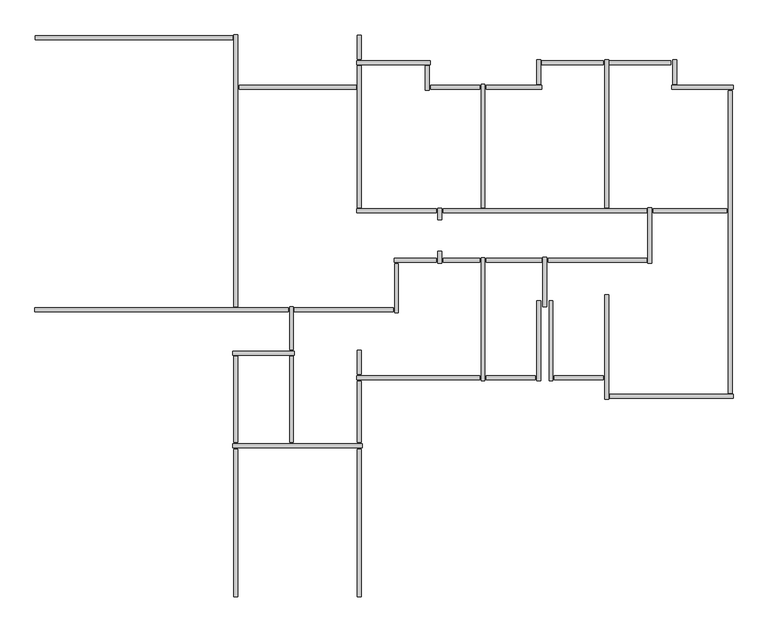
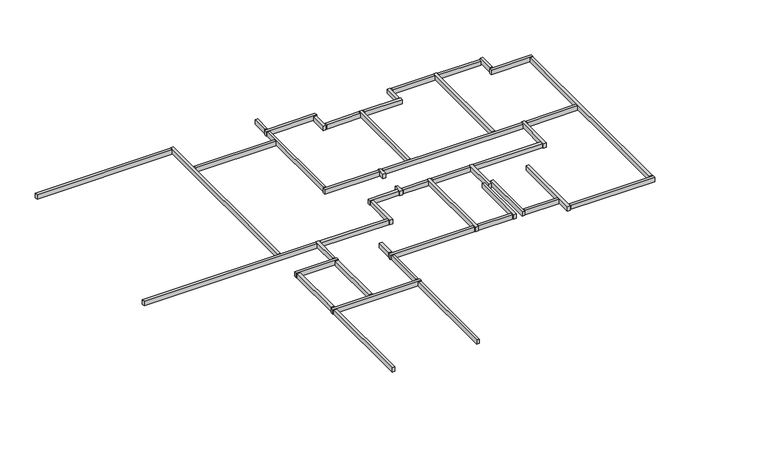
"""IFC4 building model written with IfcOpenShell, lengths in millimetres: beam geometry, Graute viga de respaldo1 : Graute viga de respaldo."""

from ifc_helpers import new_model, si_unit, frame, origin, place, context, project, spatial, polyline, outline, extrude, source, transform, mapped, element, save


def beam_8978719d(model_context):
    return source(origin(), model_context, "Body", "SweptSolid", [
        extrude(outline(polyline([(-62804.9587292, 72814.9577736), (-62804.9587292, 72720.9577736), (-67594.9587292, 72720.9577736), (-67594.9587292, 72814.9577736), (-62804.9587292, 72814.9577736)])), frame((0.0, 0.0, 2632.9999999), z_axis=(0.0, 0.0, 1.0), x_axis=(1.0, 0.0, 0.0)), (0.0, 0.0, 1.0), 167.0),
        extrude(outline(polyline([(-59771.9587292, 62785.4278788), (-59677.9587292, 62785.4278788), (-59677.9587292, 59195.4278788), (-59771.9587292, 59195.4278788), (-59771.9587292, 62785.4278788)])), frame((0.0, 0.0, 2632.9999999), z_axis=(0.0, 0.0, 1.0), x_axis=(1.0, 0.0, 0.0)), (0.0, 0.0, 1.0), 167.0),
        extrude(outline(polyline([(-62771.9587292, 62785.4278788), (-62677.9587292, 62785.4278788), (-62677.9587292, 59195.4278788), (-62771.9587292, 59195.4278788), (-62771.9587292, 62785.4278788)])), frame((0.0, 0.0, 2632.9999999), z_axis=(0.0, 0.0, 1.0), x_axis=(1.0, 0.0, 0.0)), (0.0, 0.0, 1.0), 167.0),
        extrude(outline(polyline([(-54994.9587292, 64468.4278788), (-54994.9587292, 64562.4278788), (-53804.9587292, 64562.4278788), (-53804.9587292, 64468.4278788), (-54994.9587292, 64468.4278788)])), frame((0.0, 0.0, 2632.9999999), z_axis=(0.0, 0.0, 1.0), x_axis=(1.0, 0.0, 0.0)), (0.0, 0.0, 1.0), 167.0),
        extrude(outline(polyline([(-56644.9587292, 64468.4278788), (-56644.9587292, 64562.4278788), (-55454.9587292, 64562.4278788), (-55454.9587292, 64468.4278788), (-56644.9587292, 64468.4278788)])), frame((0.0, 0.0, 2632.9999999), z_axis=(0.0, 0.0, 1.0), x_axis=(1.0, 0.0, 0.0)), (0.0, 0.0, 1.0), 167.0),
        extrude(outline(polyline([(-52594.9587292, 68518.4278788), (-52594.9587292, 68612.4278788), (-50804.9587292, 68612.4278788), (-50804.9587292, 68518.4278788), (-52594.9587292, 68518.4278788)])), frame((0.0, 0.0, 2632.9999999), z_axis=(0.0, 0.0, 1.0), x_axis=(1.0, 0.0, 0.0)), (0.0, 0.0, 1.0), 167.0),
        extrude(outline(polyline([(-57994.9587292, 71518.4278788), (-57994.9587292, 71612.4278788), (-56804.9587292, 71612.4278788), (-56804.9587292, 71518.4278788), (-57994.9587292, 71518.4278788)])), frame((0.0, 0.0, 2632.9999999), z_axis=(0.0, 0.0, 1.0), x_axis=(1.0, 0.0, 0.0)), (0.0, 0.0, 1.0), 167.0),
        extrude(outline(polyline([(-58027.9587292, 71495.4278788), (-58121.9587292, 71495.4278788), (-58121.9587292, 72085.4278788), (-58027.9587292, 72085.4278788), (-58027.9587292, 71495.4278788)])), frame((0.0, 0.0, 2632.9999999), z_axis=(0.0, 0.0, 1.0), x_axis=(1.0, 0.0, 0.0)), (0.0, 0.0, 1.0), 167.0),
        extrude(outline(polyline([(-59794.9587292, 72118.4278788), (-59794.9587292, 72212.4278788), (-58004.9587292, 72212.4278788), (-58004.9587292, 72118.4278788), (-59794.9587292, 72118.4278788)])), frame((0.0, 0.0, 2632.9999999), z_axis=(0.0, 0.0, 1.0), x_axis=(1.0, 0.0, 0.0)), (0.0, 0.0, 1.0), 167.0),
        extrude(outline(polyline([(-57821.9587292, 68635.4278788), (-57727.9587292, 68635.4278788), (-57727.9587292, 68345.4278788), (-57821.9587292, 68345.4278788), (-57821.9587292, 68635.4278788)])), frame((0.0, 0.0, 2632.9999999), z_axis=(0.0, 0.0, 1.0), x_axis=(1.0, 0.0, 0.0)), (0.0, 0.0, 1.0), 167.0),
        extrude(outline(polyline([(-55144.9587292, 67318.4278788), (-55144.9587292, 67412.4278788), (-52754.9587292, 67412.4278788), (-52754.9587292, 67318.4278788), (-55144.9587292, 67318.4278788)])), frame((0.0, 0.0, 2632.9999999), z_axis=(0.0, 0.0, 1.0), x_axis=(1.0, 0.0, 0.0)), (0.0, 0.0, 1.0), 167.0),
        extrude(outline(polyline([(-56644.9587292, 67318.4278788), (-56644.9587292, 67412.4278788), (-55304.9587292, 67412.4278788), (-55304.9587292, 67318.4278788), (-56644.9587292, 67318.4278788)])), frame((0.0, 0.0, 2632.9999999), z_axis=(0.0, 0.0, 1.0), x_axis=(1.0, 0.0, 0.0)), (0.0, 0.0, 1.0), 167.0),
        extrude(outline(polyline([(-57694.9587292, 67318.4278788), (-57694.9587292, 67412.4278788), (-56804.9587292, 67412.4278788), (-56804.9587292, 67318.4278788), (-57694.9587292, 67318.4278788)])), frame((0.0, 0.0, 2632.9999999), z_axis=(0.0, 0.0, 1.0), x_axis=(1.0, 0.0, 0.0)), (0.0, 0.0, 1.0), 167.0),
        extrude(outline(polyline([(-57821.9587292, 67585.4278788), (-57727.9587292, 67585.4278788), (-57727.9587292, 67295.4278788), (-57821.9587292, 67295.4278788), (-57821.9587292, 67585.4278788)])), frame((0.0, 0.0, 2632.9999999), z_axis=(0.0, 0.0, 1.0), x_axis=(1.0, 0.0, 0.0)), (0.0, 0.0, 1.0), 167.0),
        extrude(outline(polyline([(-58884.9587292, 67318.4278788), (-58884.9587292, 67412.4278788), (-57854.9587292, 67412.4278788), (-57854.9587292, 67318.4278788), (-58884.9587292, 67318.4278788)])), frame((0.0, 0.0, 2632.9999999), z_axis=(0.0, 0.0, 1.0), x_axis=(1.0, 0.0, 0.0)), (0.0, 0.0, 1.0), 167.0),
        extrude(outline(polyline([(-58777.9587292, 66095.4278788), (-58871.9587292, 66095.4278788), (-58871.9587292, 67285.4278788), (-58777.9587292, 67285.4278788), (-58777.9587292, 66095.4278788)])), frame((0.0, 0.0, 2632.9999999), z_axis=(0.0, 0.0, 1.0), x_axis=(1.0, 0.0, 0.0)), (0.0, 0.0, 1.0), 167.0),
        extrude(outline(polyline([(-61304.9587292, 66118.4278788), (-61304.9587292, 66212.4278788), (-58904.9587292, 66212.4278788), (-58904.9587292, 66118.4278788), (-61304.9587292, 66118.4278788)])), frame((0.0, 0.0, 2632.9999999), z_axis=(0.0, 0.0, 1.0), x_axis=(1.0, 0.0, 0.0)), (0.0, 0.0, 1.0), 167.0),
        extrude(outline(polyline([(-56771.9587292, 67430.4278788), (-56677.9587292, 67430.4278788), (-56677.9587292, 64445.4278788), (-56771.9587292, 64445.4278788), (-56771.9587292, 67430.4278788)])), frame((0.0, 0.0, 2632.9999999), z_axis=(0.0, 0.0, 1.0), x_axis=(1.0, 0.0, 0.0)), (0.0, 0.0, 1.0), 167.0),
        extrude(outline(polyline([(-59794.9587292, 64468.4278788), (-59794.9587292, 64562.4278788), (-56804.9587292, 64562.4278788), (-56804.9587292, 64468.4278788), (-59794.9587292, 64468.4278788)])), frame((0.0, 0.0, 2632.9999999), z_axis=(0.0, 0.0, 1.0), x_axis=(1.0, 0.0, 0.0)), (0.0, 0.0, 1.0), 167.0),
        extrude(outline(polyline([(-59771.9587292, 65185.4278788), (-59677.9587292, 65185.4278788), (-59677.9587292, 64595.4278788), (-59771.9587292, 64595.4278788), (-59771.9587292, 65185.4278788)])), frame((0.0, 0.0, 2632.9999999), z_axis=(0.0, 0.0, 1.0), x_axis=(1.0, 0.0, 0.0)), (0.0, 0.0, 1.0), 167.0),
        extrude(outline(polyline([(-59677.9587292, 62945.4278788), (-59771.9587292, 62945.4278788), (-59771.9587292, 64435.4278788), (-59677.9587292, 64435.4278788), (-59677.9587292, 62945.4278788)])), frame((0.0, 0.0, 2632.9999999), z_axis=(0.0, 0.0, 1.0), x_axis=(1.0, 0.0, 0.0)), (0.0, 0.0, 1.0), 167.0),
        extrude(outline(polyline([(-62677.9587292, 62945.4278788), (-62771.9587292, 62945.4278788), (-62771.9587292, 65035.4278788), (-62677.9587292, 65035.4278788), (-62677.9587292, 62945.4278788)])), frame((0.0, 0.0, 2632.9999999), z_axis=(0.0, 0.0, 1.0), x_axis=(1.0, 0.0, 0.0)), (0.0, 0.0, 1.0), 167.0),
        extrude(outline(polyline([(-61327.9587292, 62945.4278788), (-61421.9587292, 62945.4278788), (-61421.9587292, 65035.4278788), (-61327.9587292, 65035.4278788), (-61327.9587292, 62945.4278788)])), frame((0.0, 0.0, 2632.9999999), z_axis=(0.0, 0.0, 1.0), x_axis=(1.0, 0.0, 0.0)), (0.0, 0.0, 1.0), 167.0),
        extrude(outline(polyline([(-61421.9587292, 66235.4278788), (-61327.9587292, 66235.4278788), (-61327.9587292, 65195.4278788), (-61421.9587292, 65195.4278788), (-61421.9587292, 66235.4278788)])), frame((0.0, 0.0, 2632.9999999), z_axis=(0.0, 0.0, 1.0), x_axis=(1.0, 0.0, 0.0)), (0.0, 0.0, 1.0), 167.0),
        extrude(outline(polyline([(-62644.9587292, 71518.4278788), (-62644.9587292, 71612.4278788), (-59804.9587292, 71612.4278788), (-59804.9587292, 71518.4278788), (-62644.9587292, 71518.4278788)])), frame((0.0, 0.0, 2632.9999999), z_axis=(0.0, 0.0, 1.0), x_axis=(1.0, 0.0, 0.0)), (0.0, 0.0, 1.0), 167.0),
        extrude(outline(polyline([(-59677.9587292, 68645.4278788), (-59771.9587292, 68645.4278788), (-59771.9587292, 72085.4278788), (-59677.9587292, 72085.4278788), (-59677.9587292, 68645.4278788)])), frame((0.0, 0.0, 2632.9999999), z_axis=(0.0, 0.0, 1.0), x_axis=(1.0, 0.0, 0.0)), (0.0, 0.0, 1.0), 167.0),
        extrude(outline(polyline([(-59794.9587292, 68518.4278788), (-59794.9587292, 68612.4278788), (-57854.9587292, 68612.4278788), (-57854.9587292, 68518.4278788), (-59794.9587292, 68518.4278788)])), frame((0.0, 0.0, 2632.9999999), z_axis=(0.0, 0.0, 1.0), x_axis=(1.0, 0.0, 0.0)), (0.0, 0.0, 1.0), 167.0),
        extrude(outline(polyline([(-57694.9587292, 68518.4278788), (-57694.9587292, 68612.4278788), (-52754.9587292, 68612.4278788), (-52754.9587292, 68518.4278788), (-57694.9587292, 68518.4278788)])), frame((0.0, 0.0, 2632.9999999), z_axis=(0.0, 0.0, 1.0), x_axis=(1.0, 0.0, 0.0)), (0.0, 0.0, 1.0), 167.0),
        extrude(outline(polyline([(-56771.9587292, 71635.4278788), (-56677.9587292, 71635.4278788), (-56677.9587292, 68645.4278788), (-56771.9587292, 68645.4278788), (-56771.9587292, 71635.4278788)])), frame((0.0, 0.0, 2632.9999999), z_axis=(0.0, 0.0, 1.0), x_axis=(1.0, 0.0, 0.0)), (0.0, 0.0, 1.0), 167.0),
        extrude(outline(polyline([(-55304.9587292, 71612.4278788), (-55304.9587292, 71518.4278788), (-56644.9587292, 71518.4278788), (-56644.9587292, 71612.4278788), (-55304.9587292, 71612.4278788)])), frame((0.0, 0.0, 2632.9999999), z_axis=(0.0, 0.0, 1.0), x_axis=(1.0, 0.0, 0.0)), (0.0, 0.0, 1.0), 167.0),
        extrude(outline(polyline([(-55421.9587292, 72235.4278788), (-55327.9587292, 72235.4278788), (-55327.9587292, 71645.4278788), (-55421.9587292, 71645.4278788), (-55421.9587292, 72235.4278788)])), frame((0.0, 0.0, 2632.9999999), z_axis=(0.0, 0.0, 1.0), x_axis=(1.0, 0.0, 0.0)), (0.0, 0.0, 1.0), 167.0),
        extrude(outline(polyline([(-55294.9587292, 72118.4278788), (-55294.9587292, 72212.4278788), (-53804.9587292, 72212.4278788), (-53804.9587292, 72118.4278788), (-55294.9587292, 72118.4278788)])), frame((0.0, 0.0, 2632.9999999), z_axis=(0.0, 0.0, 1.0), x_axis=(1.0, 0.0, 0.0)), (0.0, 0.0, 1.0), 167.0),
        extrude(outline(polyline([(-52165.9809043, 72212.4278788), (-52165.9809043, 72117.4278788), (-53654.9587292, 72117.4278788), (-53654.9587292, 72212.4278788), (-52165.9809043, 72212.4278788)])), frame((0.0, 0.0, 2617.1856208), z_axis=(0.0, 0.0, 1.0), x_axis=(1.0, 0.0, 0.0)), (0.0, 0.0, 1.0), 165.0),
        extrude(outline(polyline([(-50677.9587292, 64145.4278788), (-50771.9587292, 64145.4278788), (-50771.9587292, 71485.4278788), (-50677.9587292, 71485.4278788), (-50677.9587292, 64145.4278788)])), frame((0.0, 0.0, 2632.9999999), z_axis=(0.0, 0.0, 1.0), x_axis=(1.0, 0.0, 0.0)), (0.0, 0.0, 1.0), 167.0),
        extrude(outline(polyline([(-52627.9587292, 67295.4278788), (-52721.9587292, 67295.4278788), (-52721.9587292, 68640.7810915), (-52627.9587292, 68640.7810915), (-52627.9587292, 67295.4278788)])), frame((0.0, 0.0, 2632.9999999), z_axis=(0.0, 0.0, 1.0), x_axis=(1.0, 0.0, 0.0)), (0.0, 0.0, 1.0), 167.0),
        extrude(outline(polyline([(-55177.9587292, 66245.4278788), (-55271.9587292, 66245.4278788), (-55271.9587292, 67435.4278788), (-55177.9587292, 67435.4278788), (-55177.9587292, 66245.4278788)])), frame((0.0, 0.0, 2632.9999999), z_axis=(0.0, 0.0, 1.0), x_axis=(1.0, 0.0, 0.0)), (0.0, 0.0, 1.0), 167.0),
        extrude(outline(polyline([(-55027.9587292, 64445.4278788), (-55121.9587292, 64445.4278788), (-55121.9587292, 66385.4278788), (-55027.9587292, 66385.4278788), (-55027.9587292, 64445.4278788)])), frame((0.0, 0.0, 2632.9999999), z_axis=(0.0, 0.0, 1.0), x_axis=(1.0, 0.0, 0.0)), (0.0, 0.0, 1.0), 167.0),
        extrude(outline(polyline([(-55327.9587292, 64445.4278788), (-55421.9587292, 64445.4278788), (-55421.9587292, 66385.4278788), (-55327.9587292, 66385.4278788), (-55327.9587292, 64445.4278788)])), frame((0.0, 0.0, 2632.9999999), z_axis=(0.0, 0.0, 1.0), x_axis=(1.0, 0.0, 0.0)), (0.0, 0.0, 1.0), 167.0),
        extrude(outline(polyline([(-53677.9587292, 63995.4278788), (-53771.9587292, 63995.4278788), (-53771.9587292, 66535.4278788), (-53677.9587292, 66535.4278788), (-53677.9587292, 63995.4278788)])), frame((0.0, 0.0, 2632.9999999), z_axis=(0.0, 0.0, 1.0), x_axis=(1.0, 0.0, 0.0)), (0.0, 0.0, 1.0), 167.0),
        extrude(outline(polyline([(-50654.9587292, 64112.4278788), (-50654.9587292, 64018.4278788), (-53644.9587292, 64018.4278788), (-53644.9587292, 64112.4278788), (-50654.9587292, 64112.4278788)])), frame((0.0, 0.0, 2632.9999999), z_axis=(0.0, 0.0, 1.0), x_axis=(1.0, 0.0, 0.0)), (0.0, 0.0, 1.0), 167.0),
        extrude(outline(polyline([(-52121.9587292, 72235.4278788), (-52027.9587292, 72235.4278788), (-52027.9587292, 71645.4278788), (-52121.9587292, 71645.4278788), (-52121.9587292, 72235.4278788)])), frame((0.0, 0.0, 2632.9999999), z_axis=(0.0, 0.0, 1.0), x_axis=(1.0, 0.0, 0.0)), (0.0, 0.0, 1.0), 167.0),
        extrude(outline(polyline([(-52144.9587292, 71518.4278788), (-52144.9587292, 71612.4278788), (-50654.9587292, 71612.4278788), (-50654.9587292, 71518.4278788), (-52144.9587292, 71518.4278788)])), frame((0.0, 0.0, 2632.9999999), z_axis=(0.0, 0.0, 1.0), x_axis=(1.0, 0.0, 0.0)), (0.0, 0.0, 1.0), 167.0),
        extrude(outline(polyline([(-53771.9587292, 72235.4278788), (-53677.9587292, 72235.4278788), (-53677.9587292, 68645.4278788), (-53771.9587292, 68645.4278788), (-53771.9587292, 72235.4278788)])), frame((0.0, 0.0, 2632.9999999), z_axis=(0.0, 0.0, 1.0), x_axis=(1.0, 0.0, 0.0)), (0.0, 0.0, 1.0), 167.0),
        extrude(outline(polyline([(-59771.9587292, 72835.4278788), (-59677.9587292, 72835.4278788), (-59677.9587292, 72245.4278788), (-59771.9587292, 72245.4278788), (-59771.9587292, 72835.4278788)])), frame((0.0, 0.0, 2632.9999999), z_axis=(0.0, 0.0, 1.0), x_axis=(1.0, 0.0, 0.0)), (0.0, 0.0, 1.0), 167.0),
        extrude(outline(polyline([(-62794.9587292, 65068.4278788), (-62794.9587292, 65162.4278788), (-61304.9587292, 65162.4278788), (-61304.9587292, 65068.4278788), (-62794.9587292, 65068.4278788)])), frame((0.0, 0.0, 2632.9999999), z_axis=(0.0, 0.0, 1.0), x_axis=(1.0, 0.0, 0.0)), (0.0, 0.0, 1.0), 167.0),
        extrude(outline(polyline([(-62794.9587292, 62818.4278788), (-62794.9587292, 62912.4278788), (-59654.9587292, 62912.4278788), (-59654.9587292, 62818.4278788), (-62794.9587292, 62818.4278788)])), frame((0.0, 0.0, 2632.9999999), z_axis=(0.0, 0.0, 1.0), x_axis=(1.0, 0.0, 0.0)), (0.0, 0.0, 1.0), 167.0),
        extrude(outline(polyline([(-67601.7587292, 66118.4278788), (-67601.7587292, 66212.4278788), (-61454.9587292, 66212.4278788), (-61454.9587292, 66118.4278788), (-67601.7587292, 66118.4278788)])), frame((0.0, 0.0, 2632.9999999), z_axis=(0.0, 0.0, 1.0), x_axis=(1.0, 0.0, 0.0)), (0.0, 0.0, 1.0), 167.0),
        extrude(outline(polyline([(-62771.9587292, 72837.9577736), (-62677.9587292, 72837.9577736), (-62677.9587292, 66245.4278788), (-62771.9587292, 66245.4278788), (-62771.9587292, 72837.9577736)])), frame((0.0, 0.0, 2632.9999999), z_axis=(0.0, 0.0, 1.0), x_axis=(1.0, 0.0, 0.0)), (0.0, 0.0, 1.0), 167.0),
    ])


if __name__ == "__main__":
    model = new_model("IFC4")
    model_context = context("Model", 3, world=origin())
    ifc_project = project(units=[si_unit("LENGTHUNIT", "METRE", prefix="MILLI")], contexts=[model_context])
    site = spatial("IfcSite", under=ifc_project)
    building = spatial("IfcBuilding", under=site)
    placement = place(None, origin())
    beam_shape = beam_8978719d(model_context)
    element("IfcBeam", 1, ObjectType="Graute viga de respaldo1 : Graute viga de respaldo", at=placement, inside=building, context=model_context, shape_type="MappedRepresentation", body=[
        mapped(beam_shape, transform((0.0, 0.0, 0.0), x_axis=(1.0, 0.0, 0.0), y_axis=(0.0, 1.0, 0.0), z_axis=(0.0, 0.0, 1.0))),
    ])
    save(model, "model.ifc")

# Revit data of these elements
# Element 1 (IfcBeam, "Graute viga de respaldo1 : Graute viga de respaldo")
#   Materials on its faces: "Concreto, Faixa de areia/cimento"
# Materials
#   "Concreto, Faixa de areia/cimento": class "Concreto", colour RGB 127 127 127, transparency 0, Description = "Revestimento de laje de concreto", Cost = 0
